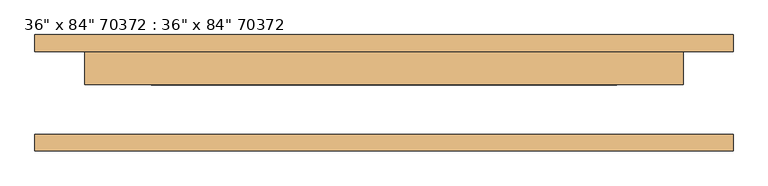
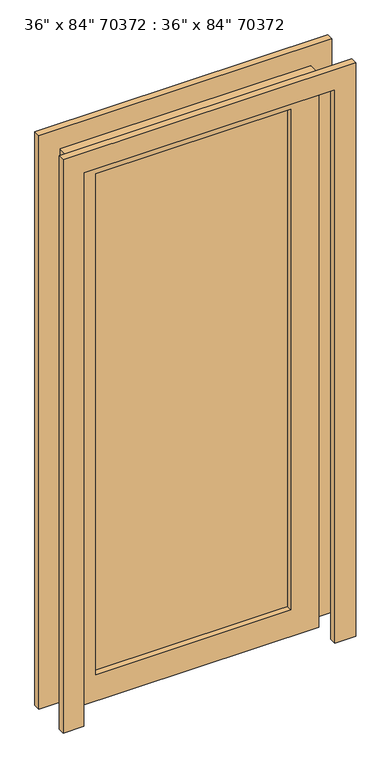
"""IFC4 building model written with IfcOpenShell, lengths in millimetres: door geometry."""

import ifcopenshell
import ifcopenshell.guid

model = None  # the IFC model being written
_history = None  # IfcOwnerHistory: only IFC2X3 demands one
_inside = {}  # id of a spatial element -> (the spatial element, [elements in it])
_under = {}  # id of a project, library or spatial element -> (it, [spatial elements below it])
_declared = {}  # id of a project -> (the project, [libraries it declares])
_typed = {}  # id of a type object -> (the type object, [elements of that type])
_made_of = {}  # id of a material, layer set ... -> (it, [elements and type objects made of it])


def new_model(schema):
    """Start an empty IFC model of exactly this schema.

    Asked for "IFC4X3", IfcOpenShell would pick the latest addendum, in which some entities
    have other attributes; the version numbers below select the first issue.
    IFC2X3 requires an IfcOwnerHistory on every rooted entity: one is made here for all.
    """
    global model, _history
    if schema == "IFC4X3":
        model = ifcopenshell.file(schema_version=(4, 3, 0, 0))
    else:
        model = ifcopenshell.file(schema=schema)
    _inside.clear()
    _under.clear()
    _declared.clear()
    _typed.clear()
    _made_of.clear()
    _history = None
    if model.schema == "IFC2X3":
        org = make("IfcOrganization", Name="unknown")
        user = make(
            "IfcPersonAndOrganization",
            ThePerson=make("IfcPerson", FamilyName="unknown"),
            TheOrganization=org,
        )
        app = make(
            "IfcApplication",
            ApplicationDeveloper=org,
            Version="unknown",
            ApplicationFullName="unknown",
            ApplicationIdentifier="unknown",
        )
        _history = make(
            "IfcOwnerHistory",
            OwningUser=user,
            OwningApplication=app,
            ChangeAction="ADDED",
            CreationDate=0,
        )
    return model


def make(cls, **values):
    """One entity of the class cls with the attributes given. An attribute that is None is left unset."""
    return model.create_entity(
        cls, **{name: value for name, value in values.items() if value is not None}
    )


def rooted(cls, **values):
    """An entity with a GlobalId (a new one), such as an element, a storey or a relation."""
    return make(cls, GlobalId=ifcopenshell.guid.new(), OwnerHistory=_history, **values)


def si_unit(unit_type, name, prefix=None):
    """IfcSIUnit, for example si_unit("LENGTHUNIT", "METRE", prefix="MILLI")."""
    return make("IfcSIUnit", UnitType=unit_type, Prefix=prefix, Name=name)


def assignment(units):
    """IfcUnitAssignment: the units of a project."""
    return None if units is None else make("IfcUnitAssignment", Units=units)


def point(xyz):
    """IfcCartesianPoint."""
    return None if xyz is None else make("IfcCartesianPoint", Coordinates=xyz)


def direction(xyz):
    """IfcDirection."""
    return None if xyz is None else make("IfcDirection", DirectionRatios=xyz)


def frame(location, z_axis=None, x_axis=None):
    """IfcAxis2Placement3D, a coordinate frame: its origin and axes. An axis left out is left unset."""
    return make(
        "IfcAxis2Placement3D",
        Location=point(location),
        Axis=direction(z_axis),
        RefDirection=direction(x_axis),
    )


def origin():
    """The frame at (0, 0, 0) with its axes left unset."""
    return frame((0.0, 0.0, 0.0))


def place(relative_to, where):
    """IfcLocalPlacement: puts the frame where relative to a parent placement (None: the world)."""
    return make(
        "IfcLocalPlacement", PlacementRelTo=relative_to, RelativePlacement=where
    )


def context(
    kind, dimensions, precision=None, world=None, true_north=None, identifier=None
):
    """IfcGeometricRepresentationContext, for example the 3D "Model" context."""
    return make(
        "IfcGeometricRepresentationContext",
        ContextIdentifier=identifier,
        ContextType=kind,
        CoordinateSpaceDimension=dimensions,
        Precision=precision,
        WorldCoordinateSystem=world,
        TrueNorth=true_north,
    )


def project(units=None, contexts=None):
    """IfcProject with its units and contexts."""
    return rooted(
        "IfcProject",
        Name="project",
        RepresentationContexts=contexts,
        UnitsInContext=assignment(units),
    )


def spatial(cls, under=None, at=None, **own):
    """A site, building, storey or space (cls), placed at a placement, below another one or the project."""
    s = rooted(cls, ObjectPlacement=at, **own)
    if under is not None:
        _under.setdefault(under.id(), (under, []))[1].append(s)
    return s


def polyline(points):
    """IfcPolyline through the points."""
    return make("IfcPolyline", Points=[point(p) for p in points])


def outline(outer, holes=None, kind="AREA"):
    """IfcArbitraryClosedProfileDef: a profile drawn as a closed curve; with holes, ...WithVoids."""
    if holes is None:
        return make("IfcArbitraryClosedProfileDef", ProfileType=kind, OuterCurve=outer)
    return make(
        "IfcArbitraryProfileDefWithVoids",
        ProfileType=kind,
        OuterCurve=outer,
        InnerCurves=holes,
    )


def extrude(swept, where, along, depth):
    """IfcExtrudedAreaSolid: the profile swept, set in the frame where, extruded along a direction by depth."""
    return make(
        "IfcExtrudedAreaSolid",
        SweptArea=swept,
        Position=where,
        ExtrudedDirection=direction(along),
        Depth=depth,
    )


def shape(context_of_items, identifier, shape_type, items):
    """IfcShapeRepresentation: the items that make up one representation, for example the "Body"."""
    return make(
        "IfcShapeRepresentation",
        ContextOfItems=context_of_items,
        RepresentationIdentifier=identifier,
        RepresentationType=shape_type,
        Items=items,
    )


def source(mapping_origin, context_of_items, identifier, shape_type, items):
    """IfcRepresentationMap: a shape defined once, which mapped items show again and again."""
    return make(
        "IfcRepresentationMap",
        MappingOrigin=mapping_origin,
        MappedRepresentation=shape(context_of_items, identifier, shape_type, items),
    )


def transform(
    local_origin,
    x_axis=None,
    y_axis=None,
    z_axis=None,
    scale=None,
    scale2=None,
    scale3=None,
    uniform=True,
):
    """IfcCartesianTransformationOperator3D, or its non-uniform kind. x_axis, y_axis, z_axis: its Axis1, 2, 3."""
    if uniform:
        return make(
            "IfcCartesianTransformationOperator3D",
            Axis1=direction(x_axis),
            Axis2=direction(y_axis),
            LocalOrigin=point(local_origin),
            Scale=scale,
            Axis3=direction(z_axis),
        )
    return make(
        "IfcCartesianTransformationOperator3DnonUniform",
        Axis1=direction(x_axis),
        Axis2=direction(y_axis),
        LocalOrigin=point(local_origin),
        Scale=scale,
        Axis3=direction(z_axis),
        Scale2=scale2,
        Scale3=scale3,
    )


def mapped(mapping_source, mapping_target):
    """IfcMappedItem: shows the shape of a source again, moved by a transform."""
    return make(
        "IfcMappedItem", MappingSource=mapping_source, MappingTarget=mapping_target
    )


def made_of(thing, what):
    """Note that an element or type object is made of a material, layer set ...; save() writes the relation."""
    if what is not None:
        _made_of.setdefault(what.id(), (what, []))[1].append(thing)
    return thing


def element(
    cls,
    number,
    at=None,
    inside=None,
    cuts=None,
    type_object=None,
    material=None,
    context=None,
    identifier="Body",
    shape_type=None,
    held_by="IfcProductDefinitionShape",
    body=None,
    shapes=None,
    **own,
):
    """One element of the class cls, such as IfcWall. Its Tag is "e" and its number.

    at: its placement. inside: the storey or other place that contains it. cuts: it is an
    opening in that element (IfcRelVoidsElement). A single representation is given by context,
    identifier, shape_type and body (its items); several are given by shapes. held_by: the class
    of the entity that holds the representations. save() writes the other relations.
    """
    e = rooted(cls, Tag="e%d" % number, ObjectPlacement=at, **own)
    if body is not None:
        shapes = [shape(context, identifier, shape_type, body)]
    if shapes is not None:
        e.Representation = make(held_by, Representations=shapes)
    if inside is not None:
        _inside.setdefault(inside.id(), (inside, []))[1].append(e)
    if cuts is not None:
        rooted(
            "IfcRelVoidsElement", RelatingBuildingElement=cuts, RelatedOpeningElement=e
        )
    if type_object is not None:
        _typed.setdefault(type_object.id(), (type_object, []))[1].append(e)
    return made_of(e, material)


def aggregate(whole, parts):
    """IfcRelAggregates: a whole, such as a stair, and the parts it consists of."""
    return rooted("IfcRelAggregates", RelatingObject=whole, RelatedObjects=parts)


def save(model, path):
    """Write the relations noted so far, then the file.

    IfcRelAggregates (storeys below a building ...), IfcRelContainedInSpatialStructure (elements
    in a storey), IfcRelDefinesByType, IfcRelAssociatesMaterial and IfcRelDeclares: one each for
    every whole, place, type object, material and project.
    """
    for whole, parts in _under.values():
        aggregate(whole, parts)
    for where, things in _inside.values():
        rooted(
            "IfcRelContainedInSpatialStructure",
            RelatedElements=things,
            RelatingStructure=where,
        )
    for kind, things in _typed.values():
        rooted("IfcRelDefinesByType", RelatedObjects=things, RelatingType=kind)
    for what, things in _made_of.values():
        rooted("IfcRelAssociatesMaterial", RelatedObjects=things, RelatingMaterial=what)
    for by, libraries in _declared.values():
        rooted("IfcRelDeclares", RelatingContext=by, RelatedDefinitions=libraries)
    model.write(path)


def door_b0d9c261(model_context):
    return source(origin(), model_context, "Body", "SweptSolid", [
        extrude(outline(polyline([(2133.6, -457.2), (2133.6, 457.2), (0.0, 457.2), (0.0, 533.4), (2209.8, 533.4), (2209.8, -533.4), (0.0, -533.4), (0.0, -457.2), (2133.6, -457.2)])), frame((0.0, -88.9, 0.0), z_axis=(0.0, 1.0, 0.0), x_axis=(0.0, 0.0, 1.0)), (0.0, 0.0, 1.0), 25.4),
        extrude(outline(polyline([(2133.6, -457.2), (2133.6, 457.2), (0.0, 457.2), (0.0, 533.4), (2209.8, 533.4), (2209.8, -533.4), (0.0, -533.4), (0.0, -457.2), (2133.6, -457.2)])), frame((0.0, 63.5, 0.0), z_axis=(0.0, 1.0, 0.0), x_axis=(0.0, 0.0, 1.0)), (0.0, 0.0, 1.0), 25.4),
        extrude(outline(polyline([(355.6, 41.275), (355.6, 34.925), (-355.6, 34.925), (-355.6, 41.275), (355.6, 41.275)])), frame((0.0, 0.0, 101.6), z_axis=(0.0, 0.0, 1.0), x_axis=(1.0, 0.0, 0.0)), (0.0, 0.0, 1.0), 1930.4),
        extrude(outline(polyline([(2133.6, -457.2), (0.0, -457.2), (0.0, 457.2), (2133.6, 457.2), (2133.6, -457.2)]), holes=[polyline([(2032.0, 355.6), (101.6, 355.6), (101.6, -355.6), (2032.0, -355.6), (2032.0, 355.6)])]), frame((0.0, 12.7, 0.0), z_axis=(0.0, 1.0, 0.0), x_axis=(0.0, 0.0, 1.0)), (0.0, 0.0, 1.0), 50.8),
    ])


if __name__ == "__main__":
    model = new_model("IFC4")
    model_context = context("Model", 3, world=origin())
    ifc_project = project(units=[si_unit("LENGTHUNIT", "METRE", prefix="MILLI")], contexts=[model_context])
    site = spatial("IfcSite", under=ifc_project)
    building = spatial("IfcBuilding", under=site)
    placement = place(None, origin())
    door_shape = door_b0d9c261(model_context)
    element("IfcDoor", 1, ObjectType="36\" x 84\" 70372 : 36\" x 84\" 70372", at=placement, inside=building, context=model_context, shape_type="MappedRepresentation", body=[
        mapped(door_shape, transform((0.0, 0.0, 0.0), x_axis=(1.0, 0.0, 0.0), y_axis=(0.0, 1.0, 0.0), z_axis=(0.0, 0.0, 1.0))),
    ])
    save(model, "model.ifc")

# Revit data of these elements
# Type "36\" x 84\" 70372 : 36\" x 84\" 70372"
#   Type IfcGUID = "0MuvbwA9n44vt4gtWSRz3A"
#   Type Mark = "11"
#   Operation = "SINGLE_SWING_LEFT"
#   NameOverride = "36\" x 84\" 70372:36\" x 84\" 70372:302034"
#   ObjectTypeOverride = "36\" x 84\" 70372"
#   Tag = "302034"
#   Reference = "36\" x 84\""
#   ThermalTransmittance = 3.7021 (stored number, unit not read)
#   IsExternal = no
